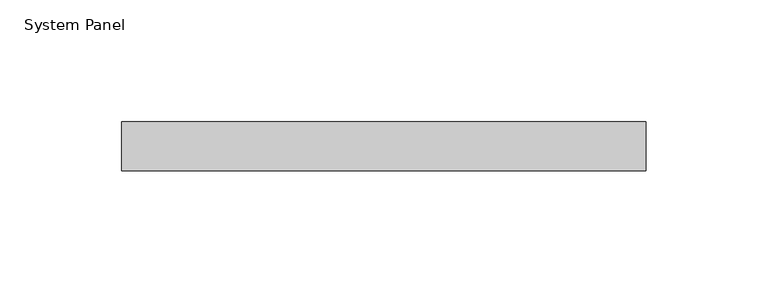
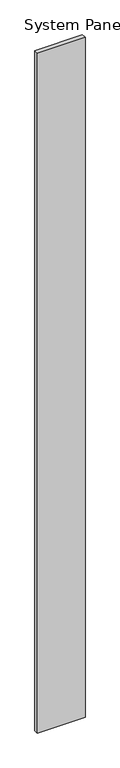
"""IFC4 building model written with IfcOpenShell, lengths in millimetres: plate geometry, System Panel : WWm-Glass-20mm-10mmOffset."""

from ifc_helpers import new_model, si_unit, origin, origin_with_axes, place, context, project, spatial, polyline, outline, extrude, source, transform, mapped, element, save


def system_panel_9caee318(model_context):
    return source(origin(), model_context, "Body", "SweptSolid", [
        extrude(outline(polyline([(107.5, 0.0), (-107.5, 0.0), (-107.5, 20.0), (107.5, 20.0), (107.5, 0.0)])), origin_with_axes(), (0.0, 0.0, 1.0), 3250.0),
    ])


if __name__ == "__main__":
    model = new_model("IFC4")
    model_context = context("Model", 3, world=origin())
    ifc_project = project(units=[si_unit("LENGTHUNIT", "METRE", prefix="MILLI")], contexts=[model_context])
    site = spatial("IfcSite", under=ifc_project)
    building = spatial("IfcBuilding", under=site)
    placement = place(None, origin())
    system_panel_shape = system_panel_9caee318(model_context)
    element("IfcPlate", 1, ObjectType="System Panel : WWm-Glass-20mm-10mmOffset", at=placement, inside=building, context=model_context, shape_type="MappedRepresentation", body=[
        mapped(system_panel_shape, transform((0.0, 0.0, 0.0), x_axis=(1.0, 0.0, 0.0), y_axis=(0.0, 1.0, 0.0), z_axis=(0.0, 0.0, 1.0))),
    ])
    save(model, "model.ifc")

# Revit data of these elements
# Type "System Panel : WWm-Glass-20mm-10mmOffset"
#   Finish = ""
# Element 1 (IfcPlate, "System Panel : WWm-Glass-20mm-10mmOffset")
#   Materials on its faces: "WW-EC-GL-Storefront"
# Materials
#   "WW-EC-GL-Storefront": class "Glass", colour RGB 236 240 239, transparency 0.85, Description = "Storefront Glass", Cost = 0
